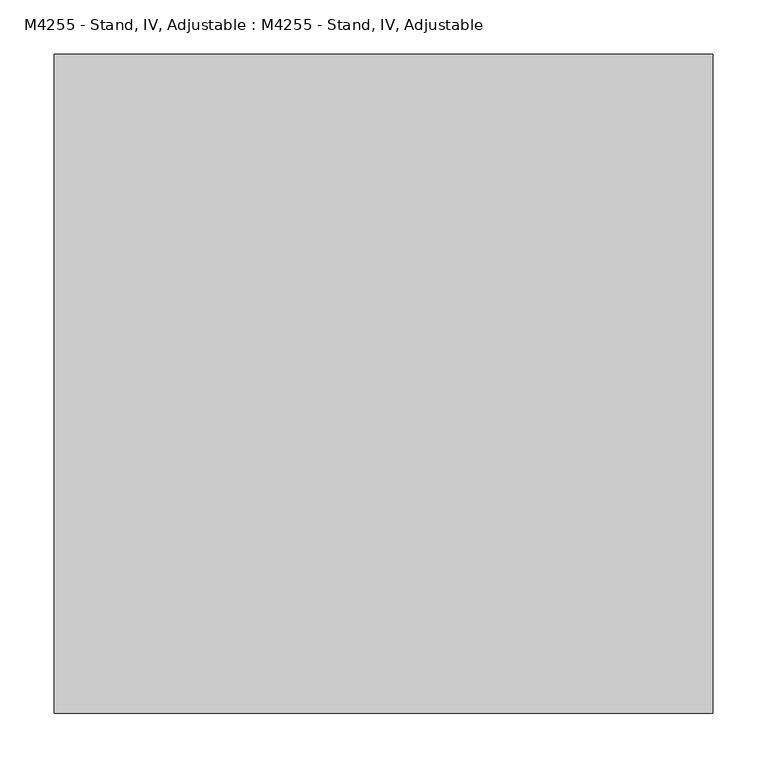
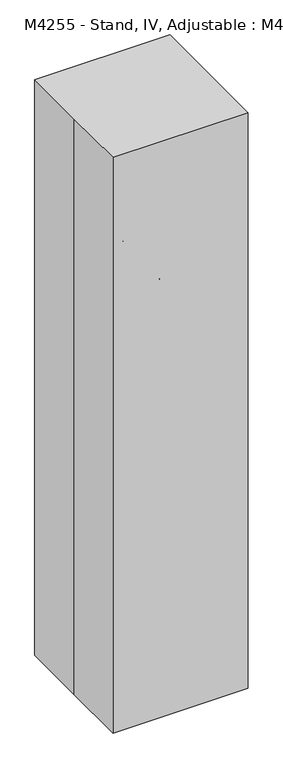
"""IFC4 building model written with IfcOpenShell, lengths in millimetres: proxy geometry, M4255 - Stand, IV, Adjustable : M4255 - Stand, IV, Adjustable."""

import ifcopenshell
import ifcopenshell.guid

model = None  # the IFC model being written
_history = None  # IfcOwnerHistory: only IFC2X3 demands one
_inside = {}  # id of a spatial element -> (the spatial element, [elements in it])
_under = {}  # id of a project, library or spatial element -> (it, [spatial elements below it])
_declared = {}  # id of a project -> (the project, [libraries it declares])
_typed = {}  # id of a type object -> (the type object, [elements of that type])
_made_of = {}  # id of a material, layer set ... -> (it, [elements and type objects made of it])


def new_model(schema):
    """Start an empty IFC model of exactly this schema.

    Asked for "IFC4X3", IfcOpenShell would pick the latest addendum, in which some entities
    have other attributes; the version numbers below select the first issue.
    IFC2X3 requires an IfcOwnerHistory on every rooted entity: one is made here for all.
    """
    global model, _history
    if schema == "IFC4X3":
        model = ifcopenshell.file(schema_version=(4, 3, 0, 0))
    else:
        model = ifcopenshell.file(schema=schema)
    _inside.clear()
    _under.clear()
    _declared.clear()
    _typed.clear()
    _made_of.clear()
    _history = None
    if model.schema == "IFC2X3":
        org = make("IfcOrganization", Name="unknown")
        user = make(
            "IfcPersonAndOrganization",
            ThePerson=make("IfcPerson", FamilyName="unknown"),
            TheOrganization=org,
        )
        app = make(
            "IfcApplication",
            ApplicationDeveloper=org,
            Version="unknown",
            ApplicationFullName="unknown",
            ApplicationIdentifier="unknown",
        )
        _history = make(
            "IfcOwnerHistory",
            OwningUser=user,
            OwningApplication=app,
            ChangeAction="ADDED",
            CreationDate=0,
        )
    return model


def make(cls, **values):
    """One entity of the class cls with the attributes given. An attribute that is None is left unset."""
    return model.create_entity(
        cls, **{name: value for name, value in values.items() if value is not None}
    )


def rooted(cls, **values):
    """An entity with a GlobalId (a new one), such as an element, a storey or a relation."""
    return make(cls, GlobalId=ifcopenshell.guid.new(), OwnerHistory=_history, **values)


def si_unit(unit_type, name, prefix=None):
    """IfcSIUnit, for example si_unit("LENGTHUNIT", "METRE", prefix="MILLI")."""
    return make("IfcSIUnit", UnitType=unit_type, Prefix=prefix, Name=name)


def assignment(units):
    """IfcUnitAssignment: the units of a project."""
    return None if units is None else make("IfcUnitAssignment", Units=units)


def point(xyz):
    """IfcCartesianPoint."""
    return None if xyz is None else make("IfcCartesianPoint", Coordinates=xyz)


def direction(xyz):
    """IfcDirection."""
    return None if xyz is None else make("IfcDirection", DirectionRatios=xyz)


def frame(location, z_axis=None, x_axis=None):
    """IfcAxis2Placement3D, a coordinate frame: its origin and axes. An axis left out is left unset."""
    return make(
        "IfcAxis2Placement3D",
        Location=point(location),
        Axis=direction(z_axis),
        RefDirection=direction(x_axis),
    )


def frame_2d(location, x_axis=None):
    """IfcAxis2Placement2D, a coordinate frame in the plane: its origin and x axis."""
    return make(
        "IfcAxis2Placement2D", Location=point(location), RefDirection=direction(x_axis)
    )


def origin():
    """The frame at (0, 0, 0) with its axes left unset."""
    return frame((0.0, 0.0, 0.0))


def origin_with_axes():
    """The frame at (0, 0, 0) with the z axis (0, 0, 1) and the x axis (1, 0, 0) written out."""
    return frame((0.0, 0.0, 0.0), z_axis=(0.0, 0.0, 1.0), x_axis=(1.0, 0.0, 0.0))


def origin_2d():
    """The frame at (0, 0) in the plane with its x axis left unset."""
    return frame_2d((0.0, 0.0))


def place(relative_to, where):
    """IfcLocalPlacement: puts the frame where relative to a parent placement (None: the world)."""
    return make(
        "IfcLocalPlacement", PlacementRelTo=relative_to, RelativePlacement=where
    )


def context(
    kind, dimensions, precision=None, world=None, true_north=None, identifier=None
):
    """IfcGeometricRepresentationContext, for example the 3D "Model" context."""
    return make(
        "IfcGeometricRepresentationContext",
        ContextIdentifier=identifier,
        ContextType=kind,
        CoordinateSpaceDimension=dimensions,
        Precision=precision,
        WorldCoordinateSystem=world,
        TrueNorth=true_north,
    )


def project(units=None, contexts=None):
    """IfcProject with its units and contexts."""
    return rooted(
        "IfcProject",
        Name="project",
        RepresentationContexts=contexts,
        UnitsInContext=assignment(units),
    )


def spatial(cls, under=None, at=None, **own):
    """A site, building, storey or space (cls), placed at a placement, below another one or the project."""
    s = rooted(cls, ObjectPlacement=at, **own)
    if under is not None:
        _under.setdefault(under.id(), (under, []))[1].append(s)
    return s


def polyline(points):
    """IfcPolyline through the points."""
    return make("IfcPolyline", Points=[point(p) for p in points])


def circle_curve(where, radius):
    """IfcCircle in the frame where."""
    return make("IfcCircle", Position=where, Radius=radius)


def ellipse_curve(where, semi_axis1, semi_axis2):
    """IfcEllipse in the frame where."""
    return make(
        "IfcEllipse", Position=where, SemiAxis1=semi_axis1, SemiAxis2=semi_axis2
    )


def trimmed(basis, trim1, trim2, sense, master):
    """IfcTrimmedCurve: the piece of a basis curve between two trims."""
    return make(
        "IfcTrimmedCurve",
        BasisCurve=basis,
        Trim1=trim1,
        Trim2=trim2,
        SenseAgreement=sense,
        MasterRepresentation=master,
    )


def segment(curve, same_sense, transition):
    """IfcCompositeCurveSegment."""
    return make(
        "IfcCompositeCurveSegment",
        Transition=transition,
        SameSense=same_sense,
        ParentCurve=curve,
    )


def composite_curve(segments, self_intersect=None):
    """IfcCompositeCurve: segments joined end to end."""
    return make("IfcCompositeCurve", Segments=segments, SelfIntersect=self_intersect)


def outline(outer, holes=None, kind="AREA"):
    """IfcArbitraryClosedProfileDef: a profile drawn as a closed curve; with holes, ...WithVoids."""
    if holes is None:
        return make("IfcArbitraryClosedProfileDef", ProfileType=kind, OuterCurve=outer)
    return make(
        "IfcArbitraryProfileDefWithVoids",
        ProfileType=kind,
        OuterCurve=outer,
        InnerCurves=holes,
    )


def extrude(swept, where, along, depth):
    """IfcExtrudedAreaSolid: the profile swept, set in the frame where, extruded along a direction by depth."""
    return make(
        "IfcExtrudedAreaSolid",
        SweptArea=swept,
        Position=where,
        ExtrudedDirection=direction(along),
        Depth=depth,
    )


def shape(context_of_items, identifier, shape_type, items):
    """IfcShapeRepresentation: the items that make up one representation, for example the "Body"."""
    return make(
        "IfcShapeRepresentation",
        ContextOfItems=context_of_items,
        RepresentationIdentifier=identifier,
        RepresentationType=shape_type,
        Items=items,
    )


def source(mapping_origin, context_of_items, identifier, shape_type, items):
    """IfcRepresentationMap: a shape defined once, which mapped items show again and again."""
    return make(
        "IfcRepresentationMap",
        MappingOrigin=mapping_origin,
        MappedRepresentation=shape(context_of_items, identifier, shape_type, items),
    )


def transform(
    local_origin,
    x_axis=None,
    y_axis=None,
    z_axis=None,
    scale=None,
    scale2=None,
    scale3=None,
    uniform=True,
):
    """IfcCartesianTransformationOperator3D, or its non-uniform kind. x_axis, y_axis, z_axis: its Axis1, 2, 3."""
    if uniform:
        return make(
            "IfcCartesianTransformationOperator3D",
            Axis1=direction(x_axis),
            Axis2=direction(y_axis),
            LocalOrigin=point(local_origin),
            Scale=scale,
            Axis3=direction(z_axis),
        )
    return make(
        "IfcCartesianTransformationOperator3DnonUniform",
        Axis1=direction(x_axis),
        Axis2=direction(y_axis),
        LocalOrigin=point(local_origin),
        Scale=scale,
        Axis3=direction(z_axis),
        Scale2=scale2,
        Scale3=scale3,
    )


def mapped(mapping_source, mapping_target):
    """IfcMappedItem: shows the shape of a source again, moved by a transform."""
    return make(
        "IfcMappedItem", MappingSource=mapping_source, MappingTarget=mapping_target
    )


def made_of(thing, what):
    """Note that an element or type object is made of a material, layer set ...; save() writes the relation."""
    if what is not None:
        _made_of.setdefault(what.id(), (what, []))[1].append(thing)
    return thing


def element(
    cls,
    number,
    at=None,
    inside=None,
    cuts=None,
    type_object=None,
    material=None,
    context=None,
    identifier="Body",
    shape_type=None,
    held_by="IfcProductDefinitionShape",
    body=None,
    shapes=None,
    **own,
):
    """One element of the class cls, such as IfcWall. Its Tag is "e" and its number.

    at: its placement. inside: the storey or other place that contains it. cuts: it is an
    opening in that element (IfcRelVoidsElement). A single representation is given by context,
    identifier, shape_type and body (its items); several are given by shapes. held_by: the class
    of the entity that holds the representations. save() writes the other relations.
    """
    e = rooted(cls, Tag="e%d" % number, ObjectPlacement=at, **own)
    if body is not None:
        shapes = [shape(context, identifier, shape_type, body)]
    if shapes is not None:
        e.Representation = make(held_by, Representations=shapes)
    if inside is not None:
        _inside.setdefault(inside.id(), (inside, []))[1].append(e)
    if cuts is not None:
        rooted(
            "IfcRelVoidsElement", RelatingBuildingElement=cuts, RelatedOpeningElement=e
        )
    if type_object is not None:
        _typed.setdefault(type_object.id(), (type_object, []))[1].append(e)
    return made_of(e, material)


def aggregate(whole, parts):
    """IfcRelAggregates: a whole, such as a stair, and the parts it consists of."""
    return rooted("IfcRelAggregates", RelatingObject=whole, RelatedObjects=parts)


def save(model, path):
    """Write the relations noted so far, then the file.

    IfcRelAggregates (storeys below a building ...), IfcRelContainedInSpatialStructure (elements
    in a storey), IfcRelDefinesByType, IfcRelAssociatesMaterial and IfcRelDeclares: one each for
    every whole, place, type object, material and project.
    """
    for whole, parts in _under.values():
        aggregate(whole, parts)
    for where, things in _inside.values():
        rooted(
            "IfcRelContainedInSpatialStructure",
            RelatedElements=things,
            RelatingStructure=where,
        )
    for kind, things in _typed.values():
        rooted("IfcRelDefinesByType", RelatedObjects=things, RelatingType=kind)
    for what, things in _made_of.values():
        rooted("IfcRelAssociatesMaterial", RelatedObjects=things, RelatingMaterial=what)
    for by, libraries in _declared.values():
        rooted("IfcRelDeclares", RelatingContext=by, RelatedDefinitions=libraries)
    model.write(path)


def plane_surface(at):
    """IfcPlane: the flat surface through the origin of the frame at, square to its z axis."""
    return make("IfcPlane", Position=at)


def cylinder_surface(at, radius):
    """IfcCylindricalSurface: all points at the distance radius from the z axis of the frame at."""
    return make("IfcCylindricalSurface", Position=at, Radius=radius)


def revolved_surface(curve, axis_point, axis_direction):
    """IfcSurfaceOfRevolution: the curve turned about the line through axis_point along axis_direction."""
    return make(
        "IfcSurfaceOfRevolution",
        SweptCurve=make("IfcArbitraryOpenProfileDef", ProfileType="CURVE", Curve=curve),
        AxisPosition=make("IfcAxis1Placement", Location=point(axis_point), Axis=direction(axis_direction)),
    )


def advanced_brep(points, edges, surfaces, faces):
    """IfcAdvancedBrep: a solid bounded by faces that lie on surfaces and meet in shared edges.

    An edge is (start, end): straight between two places in points (the first is 0);
    or (start, end, curve); or (start, end, curve, False) where it runs against its curve.
    A face is (place in surfaces, loops), or (place, loops, False) where it looks against
    its surface's normal. A loop lists edges by number (the first is 1), with a minus sign
    where the edge is run from its end to its start. The first loop is the outer one.
    """
    corners = [point(p) for p in points]
    vertices = [make("IfcVertexPoint", VertexGeometry=c) for c in corners]
    made = []
    for start, end, *more in edges:
        made.append(
            make(
                "IfcEdgeCurve",
                EdgeStart=vertices[start],
                EdgeEnd=vertices[end],
                EdgeGeometry=more[0] if more else make("IfcPolyline", Points=[corners[start], corners[end]]),
                SameSense=more[1] if len(more) > 1 else True,
            )
        )
    hull = []
    for where, loops, *sense in faces:
        bounds = []
        for j, loop in enumerate(loops):
            ring = [make("IfcOrientedEdge", EdgeElement=made[abs(k) - 1], Orientation=k > 0) for k in loop]
            bounds.append(
                make(
                    "IfcFaceOuterBound" if j == 0 else "IfcFaceBound",
                    Bound=make("IfcEdgeLoop", EdgeList=ring),
                    Orientation=True,
                )
            )
        hull.append(make("IfcAdvancedFace", Bounds=bounds, FaceSurface=surfaces[where], SameSense=sense[0] if sense else True))
    return make("IfcAdvancedBrep", Outer=make("IfcClosedShell", CfsFaces=hull))


def m4255_stand_iv_adjustable_m4255_stand_iv_adjustable_6bb1da7f(model_context):
    return source(origin(), model_context, "Body", "SolidModel", [
        extrude(outline(composite_curve([segment(trimmed(circle_curve(frame_2d((25.4, -203.0677083)), 25.4), [point((25.4, -228.4677083))], [point((25.4, -177.6677083))], False, "CARTESIAN"), True, "CONTINUOUS"), segment(trimmed(circle_curve(frame_2d((25.4, -203.0677083)), 25.4), [point((25.4, -177.6677083))], [point((25.4, -228.4677083))], False, "CARTESIAN"), True, "CONTINUOUS")], self_intersect=False)), frame((0.0, 9.525, 0.0), z_axis=(0.0, 1.0, 0.0), x_axis=(0.0, 0.0, 1.0)), (0.0, 0.0, 1.0), 9.525),
        extrude(outline(composite_curve([segment(trimmed(circle_curve(frame_2d((25.4, -203.0677083)), 25.4), [point((25.4, -177.6677083))], [point((25.4, -228.4677083))], False, "CARTESIAN"), True, "CONTINUOUS"), segment(trimmed(circle_curve(frame_2d((25.4, -203.0677083)), 25.4), [point((25.4, -228.4677083))], [point((25.4, -177.6677083))], False, "CARTESIAN"), True, "CONTINUOUS")], self_intersect=False)), frame((0.0, -19.05, 0.0), z_axis=(0.0, 1.0, 0.0), x_axis=(0.0, 0.0, 1.0)), (0.0, 0.0, 1.0), 9.525),
        extrude(outline(composite_curve([segment(trimmed(circle_curve(frame_2d((203.0677083, 25.4)), 25.4), [point((228.4677083, 25.4))], [point((177.6677083, 25.4))], False, "CARTESIAN"), True, "CONTINUOUS"), segment(trimmed(circle_curve(frame_2d((203.0677083, 25.4)), 25.4), [point((177.6677083, 25.4))], [point((228.4677083, 25.4))], False, "CARTESIAN"), True, "CONTINUOUS")], self_intersect=False)), frame((9.525, 0.0, 0.0), z_axis=(1.0, 0.0, 0.0), x_axis=(0.0, 1.0, 0.0)), (0.0, 0.0, 1.0), 9.525),
        extrude(outline(composite_curve([segment(trimmed(circle_curve(frame_2d((203.0677083, 25.4)), 25.4), [point((177.6677083, 25.4))], [point((228.4677083, 25.4))], False, "CARTESIAN"), True, "CONTINUOUS"), segment(trimmed(circle_curve(frame_2d((203.0677083, 25.4)), 25.4), [point((228.4677083, 25.4))], [point((177.6677083, 25.4))], False, "CARTESIAN"), True, "CONTINUOUS")], self_intersect=False)), frame((-19.05, 0.0, 0.0), z_axis=(1.0, 0.0, 0.0), x_axis=(0.0, 1.0, 0.0)), (0.0, 0.0, 1.0), 9.525),
        extrude(outline(composite_curve([segment(trimmed(circle_curve(frame_2d((25.4, 203.2661458)), 25.4), [point((25.4, 177.8661458))], [point((25.4, 228.6661458))], False, "CARTESIAN"), True, "CONTINUOUS"), segment(trimmed(circle_curve(frame_2d((25.4, 203.2661458)), 25.4), [point((25.4, 228.6661458))], [point((25.4, 177.8661458))], False, "CARTESIAN"), True, "CONTINUOUS")], self_intersect=False)), frame((0.0, -19.05, 0.0), z_axis=(0.0, 1.0, 0.0), x_axis=(0.0, 0.0, 1.0)), (0.0, 0.0, 1.0), 9.525),
        extrude(outline(composite_curve([segment(trimmed(circle_curve(frame_2d((25.4, 203.2661458)), 25.4), [point((25.4, 177.8661458))], [point((25.4, 228.6661458))], False, "CARTESIAN"), True, "CONTINUOUS"), segment(trimmed(circle_curve(frame_2d((25.4, 203.2661458)), 25.4), [point((25.4, 228.6661458))], [point((25.4, 177.8661458))], False, "CARTESIAN"), True, "CONTINUOUS")], self_intersect=False)), frame((0.0, 9.525, 0.0), z_axis=(0.0, 1.0, 0.0), x_axis=(0.0, 0.0, 1.0)), (0.0, 0.0, 1.0), 9.525),
        extrude(outline(composite_curve([segment(trimmed(circle_curve(frame_2d((0.0, 211.534375)), 8.4666667), [point((-8.4666667, 211.534375))], [point((8.4666667, 211.534375))], False, "CARTESIAN"), True, "CONTINUOUS"), segment(trimmed(circle_curve(frame_2d((0.0, 211.534375)), 8.4666667), [point((8.4666667, 211.534375))], [point((-8.4666667, 211.534375))], False, "CARTESIAN"), True, "CONTINUOUS")], self_intersect=False)), frame((0.0, 0.0, 25.4), z_axis=(0.0, 0.0, 1.0), x_axis=(1.0, 0.0, 0.0)), (0.0, 0.0, 1.0), 25.4),
        extrude(outline(composite_curve([segment(trimmed(circle_curve(frame_2d((203.0677083, 25.4)), 16.9333333), [point((186.134375, 25.4))], [point((220.0010417, 25.4))], False, "CARTESIAN"), True, "CONTINUOUS"), segment(trimmed(circle_curve(frame_2d((203.0677083, 25.4)), 16.9333333), [point((220.0010417, 25.4))], [point((186.134375, 25.4))], False, "CARTESIAN"), True, "CONTINUOUS")], self_intersect=False)), frame((-9.525, 0.0, 0.0), z_axis=(1.0, 0.0, 0.0), x_axis=(0.0, 1.0, 0.0)), (0.0, 0.0, 1.0), 19.05),
        extrude(outline(composite_curve([segment(trimmed(circle_curve(frame_2d((211.7328125, 0.0)), 8.4666667), [point((211.7328125, 8.4666667))], [point((211.7328125, -8.4666667))], False, "CARTESIAN"), True, "CONTINUOUS"), segment(trimmed(circle_curve(frame_2d((211.7328125, 0.0)), 8.4666667), [point((211.7328125, -8.4666667))], [point((211.7328125, 8.4666667))], False, "CARTESIAN"), True, "CONTINUOUS")], self_intersect=False)), frame((0.0, 0.0, 25.4), z_axis=(0.0, 0.0, 1.0), x_axis=(1.0, 0.0, 0.0)), (0.0, 0.0, 1.0), 25.4),
        extrude(outline(composite_curve([segment(trimmed(circle_curve(frame_2d((25.4, 203.2661458)), 16.9333333), [point((25.4, 186.3328125))], [point((25.4, 220.1994792))], False, "CARTESIAN"), True, "CONTINUOUS"), segment(trimmed(circle_curve(frame_2d((25.4, 203.2661458)), 16.9333333), [point((25.4, 220.1994792))], [point((25.4, 186.3328125))], False, "CARTESIAN"), True, "CONTINUOUS")], self_intersect=False)), frame((0.0, -9.525, 0.0), z_axis=(0.0, 1.0, 0.0), x_axis=(0.0, 0.0, 1.0)), (0.0, 0.0, 1.0), 19.05),
        extrude(outline(composite_curve([segment(trimmed(circle_curve(frame_2d((-211.534375, 0.0)), 8.4666667), [point((-211.534375, -8.4666667))], [point((-211.534375, 8.4666667))], False, "CARTESIAN"), True, "CONTINUOUS"), segment(trimmed(circle_curve(frame_2d((-211.534375, 0.0)), 8.4666667), [point((-211.534375, 8.4666667))], [point((-211.534375, -8.4666667))], False, "CARTESIAN"), True, "CONTINUOUS")], self_intersect=False)), frame((0.0, 0.0, 25.4), z_axis=(0.0, 0.0, 1.0), x_axis=(1.0, 0.0, 0.0)), (0.0, 0.0, 1.0), 25.4),
        extrude(outline(composite_curve([segment(trimmed(circle_curve(frame_2d((25.4, -203.0677083)), 16.9333333), [point((25.4, -186.134375))], [point((25.4, -220.0010417))], False, "CARTESIAN"), True, "CONTINUOUS"), segment(trimmed(circle_curve(frame_2d((25.4, -203.0677083)), 16.9333333), [point((25.4, -220.0010417))], [point((25.4, -186.134375))], False, "CARTESIAN"), True, "CONTINUOUS")], self_intersect=False)), frame((0.0, -9.525, 0.0), z_axis=(0.0, 1.0, 0.0), x_axis=(0.0, 0.0, 1.0)), (0.0, 0.0, 1.0), 19.05),
        extrude(outline(composite_curve([segment(trimmed(circle_curve(frame_2d((-203.2165365, 25.4)), 25.4), [point((-177.8165365, 25.4))], [point((-228.6165365, 25.4))], False, "CARTESIAN"), True, "CONTINUOUS"), segment(trimmed(circle_curve(frame_2d((-203.2165365, 25.4)), 25.4), [point((-228.6165365, 25.4))], [point((-177.8165365, 25.4))], False, "CARTESIAN"), True, "CONTINUOUS")], self_intersect=False)), frame((-19.05, 0.0, 0.0), z_axis=(1.0, 0.0, 0.0), x_axis=(0.0, 1.0, 0.0)), (0.0, 0.0, 1.0), 9.525),
        extrude(outline(composite_curve([segment(trimmed(circle_curve(frame_2d((-203.2165365, 25.4)), 25.4), [point((-177.8165365, 25.4))], [point((-228.6165365, 25.4))], False, "CARTESIAN"), True, "CONTINUOUS"), segment(trimmed(circle_curve(frame_2d((-203.2165365, 25.4)), 25.4), [point((-228.6165365, 25.4))], [point((-177.8165365, 25.4))], False, "CARTESIAN"), True, "CONTINUOUS")], self_intersect=False)), frame((9.525, 0.0, 0.0), z_axis=(1.0, 0.0, 0.0), x_axis=(0.0, 1.0, 0.0)), (0.0, 0.0, 1.0), 9.525),
        extrude(outline(composite_curve([segment(trimmed(circle_curve(frame_2d((0.0, -211.6832031)), 8.4666667), [point((8.4666667, -211.6832031))], [point((-8.4666667, -211.6832031))], False, "CARTESIAN"), True, "CONTINUOUS"), segment(trimmed(circle_curve(frame_2d((0.0, -211.6832031)), 8.4666667), [point((-8.4666667, -211.6832031))], [point((8.4666667, -211.6832031))], False, "CARTESIAN"), True, "CONTINUOUS")], self_intersect=False)), frame((0.0, 0.0, 25.4), z_axis=(0.0, 0.0, 1.0), x_axis=(1.0, 0.0, 0.0)), (0.0, 0.0, 1.0), 25.4),
        extrude(outline(composite_curve([segment(trimmed(circle_curve(frame_2d((-203.2165365, 25.4)), 16.9333333), [point((-186.2832031, 25.4))], [point((-220.1498698, 25.4))], False, "CARTESIAN"), True, "CONTINUOUS"), segment(trimmed(circle_curve(frame_2d((-203.2165365, 25.4)), 16.9333333), [point((-220.1498698, 25.4))], [point((-186.2832031, 25.4))], False, "CARTESIAN"), True, "CONTINUOUS")], self_intersect=False)), frame((-9.525, 0.0, 0.0), z_axis=(1.0, 0.0, 0.0), x_axis=(0.0, 1.0, 0.0)), (0.0, 0.0, 1.0), 19.05),
        extrude(outline(polyline([(-228.6, 63.5), (-192.6166667, 63.5), (-44.45, 25.4), (44.45, 25.4), (192.6166667, 63.5), (228.6, 63.5), (228.6, 50.8), (193.8216772, 50.8), (45.6550105, 12.7), (-45.6550105, 12.7), (-193.8216772, 50.8), (-228.6, 50.8), (-228.6, 63.5)])), frame((-19.05, 0.0, 0.0), z_axis=(1.0, 0.0, 0.0), x_axis=(0.0, 1.0, 0.0)), (0.0, 0.0, 1.0), 38.1),
        extrude(outline(composite_curve([segment(trimmed(circle_curve(origin_2d(), 12.7), [point((-12.7, 0.0))], [point((12.7, 0.0))], False, "CARTESIAN"), True, "CONTINUOUS"), segment(trimmed(circle_curve(origin_2d(), 12.7), [point((12.7, 0.0))], [point((-12.7, 0.0))], False, "CARTESIAN"), True, "CONTINUOUS")], self_intersect=False)), frame((0.0, 0.0, 12.7), z_axis=(0.0, 0.0, 1.0), x_axis=(1.0, 0.0, 0.0)), (0.0, 0.0, 1.0), 1473.2),
        extrude(outline(polyline([(63.5, -228.6), (50.8, -228.6), (50.8, -193.8216772), (12.7, -45.6550105), (12.7, 45.6550105), (50.8, 193.8216772), (50.8, 228.6), (63.5, 228.6), (63.5, 192.6166667), (25.4, 44.45), (25.4, -44.45), (63.5, -192.6166667), (63.5, -228.6)])), frame((0.0, -19.05, 0.0), z_axis=(0.0, 1.0, 0.0), x_axis=(0.0, 0.0, 1.0)), (0.0, 0.0, 1.0), 38.1),
        extrude(outline(composite_curve([segment(trimmed(circle_curve(origin_2d(), 6.35), [point((-6.35, 0.0))], [point((6.35, 0.0))], False, "CARTESIAN"), True, "CONTINUOUS"), segment(trimmed(circle_curve(origin_2d(), 6.35), [point((6.35, 0.0))], [point((-6.35, 0.0))], False, "CARTESIAN"), True, "CONTINUOUS")], self_intersect=False)), frame((0.0, 0.0, 1485.9), z_axis=(0.0, 0.0, 1.0), x_axis=(1.0, 0.0, 0.0)), (0.0, 0.0, 1.0), 495.3),
        advanced_brep(
        [(0.0, 117.4754217, 1962.0563468), (0.0, 111.8996536, 1954.3338837), (0.0, 135.0535266, 1949.3646141), (0.0, 129.4777585, 1941.6421511), (0.0, 139.7, 1973.2625), (0.0, 139.7, 1963.7375), (0.0, -139.7, 1963.7375), (0.0, -139.7, 1973.2625), (0.0, -129.4777585, 1941.6421511), (0.0, -135.0535266, 1949.3646141), (0.0, -117.4754217, 1962.0563468), (0.0, -111.8996536, 1954.3338837)],
        [
            (0, 1, circle_curve(frame((0.0, 114.6875376, 1958.1951153), z_axis=(0.0, -0.8107572744902805, 0.5853824748496423), x_axis=(0.0, -0.5853824748496423, -0.8107572744902805)), 4.7625)),
            (1, 0, circle_curve(frame((0.0, 114.6875376, 1958.1951153), z_axis=(0.0, -0.8107572744902805, 0.5853824748496423), x_axis=(0.0, -0.5853824748496423, -0.8107572744902805)), 4.7625)),
            (0, 2),
            (2, 3, circle_curve(frame((0.0, 132.2656426, 1945.5033826), z_axis=(0.0, -0.8107572744902805, 0.5853824748496423), x_axis=(0.0, -0.5853824748496423, -0.8107572744902805)), 4.7625)),
            (3, 1),
            (3, 2, circle_curve(frame((0.0, 132.2656426, 1945.5033826), z_axis=(0.0, -0.8107572744902805, 0.5853824748496423), x_axis=(0.0, -0.5853824748496423, -0.8107572744902805)), 4.7625)),
            (4, 3, circle_curve(frame((0.0, 139.7, 1955.8), z_axis=(-1.0, 0.0, 0.0), x_axis=(0.0, -0.5853824748496388, -0.810757274490283)), 17.4625)),
            (2, 5, circle_curve(frame((0.0, 139.7, 1955.8), z_axis=(1.0, 0.0, 0.0), x_axis=(0.0, -0.5853824748496388, -0.810757274490283)), 7.9375)),
            (5, 4, circle_curve(frame((0.0, 139.7, 1968.5), z_axis=(0.0, 1.0, 0.0), x_axis=(0.0, 0.0, 1.0)), 4.7625)),
            (4, 5, circle_curve(frame((0.0, 139.7, 1968.5), z_axis=(0.0, 1.0, 0.0), x_axis=(0.0, 0.0, 1.0)), 4.7625)),
            (5, 6),
            (6, 7, circle_curve(frame((0.0, -139.7, 1968.5), z_axis=(0.0, 1.0, 0.0), x_axis=(0.0, 0.0, 1.0)), 4.7625)),
            (7, 4),
            (7, 6, circle_curve(frame((0.0, -139.7, 1968.5), z_axis=(0.0, 1.0, 0.0), x_axis=(0.0, 0.0, 1.0)), 4.7625)),
            (8, 7, circle_curve(frame((0.0, -139.7, 1955.8), z_axis=(-1.0, 0.0, 0.0), x_axis=(0.0, 0.0, 1.0)), 17.4625)),
            (6, 9, circle_curve(frame((0.0, -139.7, 1955.8), z_axis=(1.0, 0.0, 0.0), x_axis=(0.0, 0.0, 1.0)), 7.9375)),
            (9, 8, circle_curve(frame((0.0, -132.2656426, 1945.5033826), z_axis=(0.0, -0.8107572744906172, -0.5853824748491758), x_axis=(0.0, 0.5853824748491758, -0.8107572744906172)), 4.7625)),
            (8, 9, circle_curve(frame((0.0, -132.2656426, 1945.5033826), z_axis=(0.0, -0.8107572744895747, -0.5853824748506197), x_axis=(0.0, 0.5853824748506197, -0.8107572744895747)), 4.7625)),
            (10, 11, circle_curve(frame((0.0, -114.6875376, 1958.1951153), z_axis=(0.0, 0.8107572744898955, 0.5853824748501754), x_axis=(0.0, 0.5853824748501754, -0.8107572744898955)), 4.7625)),
            (11, 10, circle_curve(frame((0.0, -114.6875376, 1958.1951153), z_axis=(0.0, 0.8107572744898955, 0.5853824748501754), x_axis=(0.0, 0.5853824748501754, -0.8107572744898955)), 4.7625)),
            (9, 10),
            (11, 8),
        ],
        [
            plane_surface(frame((266.7, 114.6875376, 1958.1951153), z_axis=(0.0, -0.8107572744902805, 0.5853824748496423), x_axis=(-1.0, 0.0, 0.0))),
            cylinder_surface(frame((0.0, 114.6875376, 1958.1951153), z_axis=(0.0, -0.8107572744902805, 0.5853824748496423), x_axis=(0.0, -0.5853824748496423, -0.8107572744902805)), 4.7625),
            revolved_surface(trimmed(ellipse_curve(frame((0.0, 132.2656426, 1945.5033826), z_axis=(0.0, -0.810757274490283, 0.5853824748496388), x_axis=(0.0, -0.5853824748496388, -0.810757274490283)), 4.7625, 4.7625), [point((0.0, 135.0535266, 1949.3646141))], [point((0.0, 129.4777585, 1941.6421511))], True, "CARTESIAN"), (266.7, 139.7, 1955.8), (1.0, 0.0, 0.0)),
            revolved_surface(trimmed(ellipse_curve(frame((0.0, 132.2656426, 1945.5033826), z_axis=(0.0, -0.810757274490283, 0.5853824748496388), x_axis=(0.0, -0.5853824748496388, -0.810757274490283)), 4.7625, 4.7625), [point((0.0, 129.4777585, 1941.6421511))], [point((0.0, 135.0535266, 1949.3646141))], True, "CARTESIAN"), (266.7, 139.7, 1955.8), (1.0, 0.0, 0.0)),
            cylinder_surface(frame((0.0, 139.7, 1968.5), z_axis=(0.0, 1.0, 0.0), x_axis=(0.0, 0.0, 1.0)), 4.7625),
            revolved_surface(trimmed(ellipse_curve(frame((0.0, -139.7, 1968.5), z_axis=(0.0, 1.0, 0.0), x_axis=(0.0, 0.0, 1.0)), 4.7625, 4.7625), [point((0.0, -139.7, 1963.7375))], [point((0.0, -139.7, 1973.2625))], True, "CARTESIAN"), (266.7, -139.7, 1955.8), (1.0, 0.0, 0.0)),
            revolved_surface(trimmed(ellipse_curve(frame((0.0, -139.7, 1968.5), z_axis=(0.0, 1.0, 0.0), x_axis=(0.0, 0.0, 1.0)), 4.7625, 4.7625), [point((0.0, -139.7, 1973.2625))], [point((0.0, -139.7, 1963.7375))], True, "CARTESIAN"), (266.7, -139.7, 1955.8), (1.0, 0.0, 0.0)),
            plane_surface(frame((266.7, -114.6875376, 1958.1951153), z_axis=(0.0, 0.8107572744898955, 0.5853824748501754), x_axis=(-1.0, 0.0, 0.0))),
            cylinder_surface(frame((0.0, -132.2656426, 1945.5033826), z_axis=(0.0, -0.8107572744898955, -0.5853824748501754), x_axis=(0.0, 0.5853824748501754, -0.8107572744898955)), 4.7625),
        ],
        [
            (0, [[1, 2]]),
            (1, [[-1, 3, 4, 5]]),
            (1, [[-2, -5, 6, -3]]),
            (2, [[7, -4, 8, 9]]),
            (3, [[-8, -6, -7, 10]]),
            (4, [[-9, 11, 12, 13]]),
            (4, [[-10, -13, 14, -11]]),
            (5, [[15, -12, 16, 17]]),
            (6, [[-16, -14, -15, 18]]),
            (7, [[19, 20]]),
            (8, [[-17, 21, -20, 22]]),
            (8, [[-18, -22, -19, -21]]),
        ],
    ),
        advanced_brep(
        [(-117.4754217, 0.0, 1962.0563468), (-111.8996536, 0.0, 1954.3338837), (-135.0535266, 0.0, 1949.3646141), (-129.4777585, 0.0, 1941.6421511), (-139.7, 0.0, 1973.2625), (-139.7, 0.0, 1963.7375), (139.7, 0.0, 1963.7375), (139.7, 0.0, 1973.2625), (129.4777585, 0.0, 1941.6421511), (135.0535266, 0.0, 1949.3646141), (117.4754217, 0.0, 1962.0563468), (111.8996536, 0.0, 1954.3338837)],
        [
            (0, 1, circle_curve(frame((-114.6875376, 0.0, 1958.1951153), z_axis=(0.810757274490287, 0.0, 0.5853824748496333), x_axis=(0.5853824748496333, 0.0, -0.810757274490287)), 4.7625)),
            (1, 0, circle_curve(frame((-114.6875376, 0.0, 1958.1951153), z_axis=(0.810757274490287, 0.0, 0.5853824748496333), x_axis=(0.5853824748496333, 0.0, -0.810757274490287)), 4.7625)),
            (0, 2),
            (2, 3, circle_curve(frame((-132.2656426, 0.0, 1945.5033826), z_axis=(0.810757274490287, 0.0, 0.5853824748496333), x_axis=(0.5853824748496333, 0.0, -0.810757274490287)), 4.7625)),
            (3, 1),
            (3, 2, circle_curve(frame((-132.2656426, 0.0, 1945.5033826), z_axis=(0.810757274490287, 0.0, 0.5853824748496333), x_axis=(0.5853824748496333, 0.0, -0.810757274490287)), 4.7625)),
            (4, 3, circle_curve(frame((-139.7, 0.0, 1955.8), z_axis=(0.0, -1.0, 0.0), x_axis=(0.5853824748496308, 0.0, -0.8107572744902887)), 17.4625)),
            (2, 5, circle_curve(frame((-139.7, 0.0, 1955.8), z_axis=(0.0, 1.0, 0.0), x_axis=(0.5853824748496308, 0.0, -0.8107572744902887)), 7.9375)),
            (5, 4, circle_curve(frame((-139.7, 0.0, 1968.5), z_axis=(-1.0, 0.0, 0.0), x_axis=(0.0, 0.0, 1.0)), 4.7625)),
            (4, 5, circle_curve(frame((-139.7, 0.0, 1968.5), z_axis=(-1.0, 0.0, 0.0), x_axis=(0.0, 0.0, 1.0)), 4.7625)),
            (5, 6),
            (6, 7, circle_curve(frame((139.7, 0.0, 1968.5), z_axis=(-1.0, 0.0, 0.0), x_axis=(0.0, 0.0, 1.0)), 4.7625)),
            (7, 4),
            (7, 6, circle_curve(frame((139.7, 0.0, 1968.5), z_axis=(-1.0, 0.0, 0.0), x_axis=(0.0, 0.0, 1.0)), 4.7625)),
            (8, 7, circle_curve(frame((139.7, 0.0, 1955.8), z_axis=(0.0, -1.0, 0.0), x_axis=(0.0, 0.0, 1.0)), 17.4625)),
            (6, 9, circle_curve(frame((139.7, 0.0, 1955.8), z_axis=(0.0, 1.0, 0.0), x_axis=(0.0, 0.0, 1.0)), 7.9375)),
            (9, 8, circle_curve(frame((132.2656426, 0.0, 1945.5033826), z_axis=(0.8107572744899008, 0.0, -0.585382474850168), x_axis=(-0.585382474850168, 0.0, -0.8107572744899008)), 4.7625)),
            (8, 9, circle_curve(frame((132.2656426, 0.0, 1945.5033826), z_axis=(0.8107572744899039, 0.0, -0.5853824748501637), x_axis=(-0.5853824748501637, 0.0, -0.8107572744899039)), 4.7625)),
            (10, 11, circle_curve(frame((114.6875376, 0.0, 1958.1951153), z_axis=(-0.8107572744899005, 0.0, 0.5853824748501685), x_axis=(-0.5853824748501685, 0.0, -0.8107572744899005)), 4.7625)),
            (11, 10, circle_curve(frame((114.6875376, 0.0, 1958.1951153), z_axis=(-0.8107572744899005, 0.0, 0.5853824748501685), x_axis=(-0.5853824748501685, 0.0, -0.8107572744899005)), 4.7625)),
            (9, 10),
            (11, 8),
        ],
        [
            plane_surface(frame((-114.6875376, 215.9, 1958.1951153), z_axis=(0.810757274490287, 0.0, 0.5853824748496333), x_axis=(0.0, -1.0, 0.0))),
            cylinder_surface(frame((-114.6875376, 0.0, 1958.1951153), z_axis=(0.810757274490287, 0.0, 0.5853824748496333), x_axis=(0.5853824748496333, 0.0, -0.810757274490287)), 4.7625),
            revolved_surface(trimmed(ellipse_curve(frame((-132.2656426, 0.0, 1945.5033826), z_axis=(0.8107572744902886, 0.0, 0.585382474849631), x_axis=(0.585382474849631, 0.0, -0.8107572744902886)), 4.7625, 4.7625), [point((-135.0535266, 0.0, 1949.3646141))], [point((-129.4777585, 0.0, 1941.6421511))], True, "CARTESIAN"), (-139.7, 215.9, 1955.8), (0.0, 1.0, 0.0)),
            revolved_surface(trimmed(ellipse_curve(frame((-132.2656426, 0.0, 1945.5033826), z_axis=(0.8107572744902886, 0.0, 0.585382474849631), x_axis=(0.585382474849631, 0.0, -0.8107572744902886)), 4.7625, 4.7625), [point((-129.4777585, 0.0, 1941.6421511))], [point((-135.0535266, 0.0, 1949.3646141))], True, "CARTESIAN"), (-139.7, 215.9, 1955.8), (0.0, 1.0, 0.0)),
            cylinder_surface(frame((-139.7, 0.0, 1968.5), z_axis=(-1.0, 0.0, 0.0), x_axis=(0.0, 0.0, 1.0)), 4.7625),
            revolved_surface(trimmed(ellipse_curve(frame((139.7, 0.0, 1968.5), z_axis=(-1.0, 0.0, 0.0), x_axis=(0.0, 0.0, 1.0)), 4.7625, 4.7625), [point((139.7, 0.0, 1963.7375))], [point((139.7, 0.0, 1973.2625))], True, "CARTESIAN"), (139.7, 215.9, 1955.8), (0.0, 1.0, 0.0)),
            revolved_surface(trimmed(ellipse_curve(frame((139.7, 0.0, 1968.5), z_axis=(-1.0, 0.0, 0.0), x_axis=(0.0, 0.0, 1.0)), 4.7625, 4.7625), [point((139.7, 0.0, 1973.2625))], [point((139.7, 0.0, 1963.7375))], True, "CARTESIAN"), (139.7, 215.9, 1955.8), (0.0, 1.0, 0.0)),
            plane_surface(frame((114.6875376, 215.9, 1958.1951153), z_axis=(-0.8107572744899004, 0.0, 0.5853824748501686), x_axis=(0.0, -1.0, 0.0))),
            cylinder_surface(frame((132.2656426, 0.0, 1945.5033826), z_axis=(0.8107572744899005, 0.0, -0.5853824748501685), x_axis=(-0.5853824748501685, 0.0, -0.8107572744899005)), 4.7625),
        ],
        [
            (0, [[1, 2]]),
            (1, [[-1, 3, 4, 5]]),
            (1, [[-2, -5, 6, -3]]),
            (2, [[7, -4, 8, 9]]),
            (3, [[-8, -6, -7, 10]]),
            (4, [[-9, 11, 12, 13]]),
            (4, [[-10, -13, 14, -11]]),
            (5, [[15, -12, 16, 17]]),
            (6, [[-16, -14, -15, 18]]),
            (7, [[19, 20]]),
            (8, [[-17, 21, -20, 22]]),
            (8, [[-18, -22, -19, -21]]),
        ],
    ),
        extrude(outline(polyline([(-304.8, 304.8), (304.8, 304.8), (304.8, -304.8), (-304.8, -304.8), (-304.8, 0.0), (-304.8, 304.8)])), origin_with_axes(), (0.0, 0.0, 1.0), 2743.2),
    ])


if __name__ == "__main__":
    model = new_model("IFC4")
    model_context = context("Model", 3, world=origin())
    ifc_project = project(units=[si_unit("LENGTHUNIT", "METRE", prefix="MILLI")], contexts=[model_context])
    site = spatial("IfcSite", under=ifc_project)
    building = spatial("IfcBuilding", under=site)
    placement = place(None, origin())
    m4255_stand_iv_adjustable_m4255_stand_iv_adjustable_shape = m4255_stand_iv_adjustable_m4255_stand_iv_adjustable_6bb1da7f(model_context)
    element("IfcBuildingElementProxy", 1, Name="M4255 - Stand, IV, Adjustable : M4255 - Stand, IV, Adjustable", ObjectType="M4255 - Stand, IV, Adjustable : M4255 - Stand, IV, Adjustable", at=placement, inside=building, context=model_context, shape_type="MappedRepresentation", body=[
        mapped(m4255_stand_iv_adjustable_m4255_stand_iv_adjustable_shape, transform((0.0, 0.0, 0.0), x_axis=(1.0, 0.0, 0.0), y_axis=(0.0, 1.0, 0.0), z_axis=(0.0, 0.0, 1.0))),
    ])
    save(model, "model.ifc")

# Revit data of these elements
# Type "M4255 - Stand, IV, Adjustable : M4255 - Stand, IV, Adjustable"
#   Watts2 = "0"
#   Watts1 = "0"
#   Unit_Issue = "EA"
#   UTIL_6_Misc = "-"
#   UTIL_5_NonMedGas = "-"
#   UTIL_4_MiscGas = "-"
#   UTIL_3_MedGas = "-"
#   UTIL_2_Elec = "-"
#   UTIL_1_WaterDrain = "-"
#   Nomenclature = "Stand, IV, Adjustable"
#   NSN = "6530"
#   Location [instance default] = ""
#   JSN = "M4255"
#   Fund_Source_VA = "-"
#   Fund_Source_Navy = "-"
#   Fund_Source_Army = "-"
#   Fund_Source_AF = "-"
#   ELEC_Volts2 = "0"
#   ELEC_Volts1 = "0"
#   ELEC_Phase2 = "0"
#   ELEC_Phase1 = "0"
#   ELEC_HertzSwitch = "0"
#   ELEC_HertzDependent = "0"
#   ELEC_Hertz = "0"
#   ELEC_Amps2 = "0"
#   ELEC_Amps1 = "0"
#   DetailDescription = "Adjustable IV stand with 4-hook arrangement. Stand has stainless steel construction with heavy weight base. It adjusts from 66 inches to 100 inches and is mounted on conductive rubber, ball bearing, swivel casters. Stand is used for administering intravenous solutions."
#   CAT_VA = "C"
#   CAT_Navy = "C"
#   CAT_IHS = "-"
#   CAT_Army = "C"
#   CAT_AF = "C"
#   BTUperhour = "0"
#   radius = 0' - 1"
#   calc 2 = 0' - 0.33333"
#   calc 1 = 0' - 0.66667"
#   Weight_IP = 35
#   DIM_Width_IP = 2' - 0"
#   DIM_Height_IP = 9' - 0"
#   DIM_Depth_IP = 2' - 0"
#   finish [instance default] = none
# Element 1 (IfcBuildingElementProxy, "M4255 - Stand, IV, Adjustable : M4255 - Stand, IV, Adjustable")
#   Location = "TRPE1"
#   Materials on its faces: "EquipSpace"
# Materials
#   "EquipSpace": class "Unassigned", colour RGB 221 217 195, transparency 0.5
